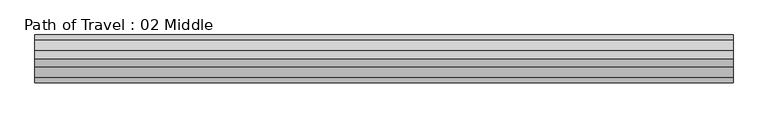
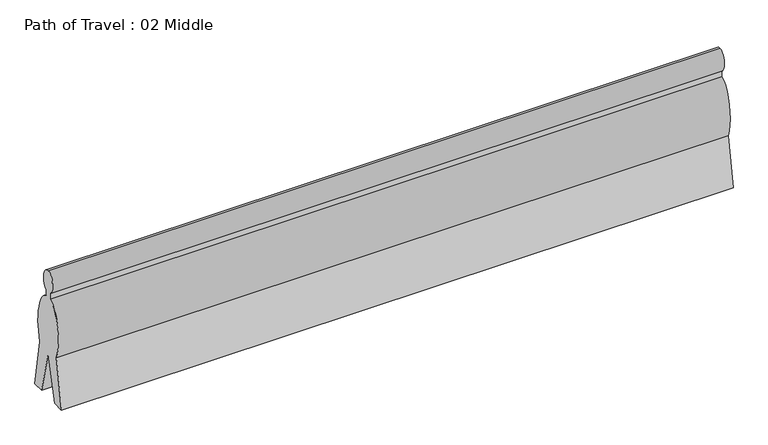
"""IFC4 building model written with IfcOpenShell, lengths in millimetres: proxy geometry, Path of Travel : 02 Middle."""

from ifc_helpers import new_model, si_unit, point, frame, origin, place, context, project, spatial, ellipse_curve, trimmed, source, transform, mapped, element, save
from ifc_brep_helpers import plane_surface, extruded_surface, advanced_brep


def path_of_travel_02_middle_3b68c140(model_context):
    return source(origin(), model_context, "Body", "AdvancedBrep", [
        advanced_brep(
        [(227.5554837, 0.0, 1727.2), (227.5554837, 42.9018657, 1436.6534209), (227.5554837, 42.9018657, 1363.4763406), (227.5554837, 184.1186263, 643.4144547), (227.5554837, 297.5699544, 0.0), (227.5554837, 145.6574193, 0.0), (227.5554837, 0.0, 584.2), (227.5554837, -145.6574193, 0.0), (227.5554837, -297.5699544, 0.0), (227.5554837, -184.1186263, 643.4144547), (227.5554837, -42.9018657, 1363.4763406), (227.5554837, -42.9018657, 1436.6534209), (8914.3554837, 0.0, 1727.2), (8914.3554837, -42.9018657, 1436.6534209), (8914.3554837, -42.9018657, 1363.4763406), (8914.3554837, -184.1186263, 643.4144547), (8914.3554837, -297.5699544, 0.0), (8914.3554837, -145.6574193, 0.0), (8914.3554837, 0.0, 584.2), (8914.3554837, 145.6574193, 0.0), (8914.3554837, 297.5699544, 0.0), (8914.3554837, 184.1186263, 643.4144547), (8914.3554837, 42.9018657, 1363.4763406), (8914.3554837, 42.9018657, 1436.6534209)],
        [
            (0, 1, ellipse_curve(frame((227.5554837, 0.0, 1574.8), z_axis=(-1.0, 0.0, 0.0), x_axis=(0.0, 0.0, 1.0)), 152.4, 101.6)),
            (1, 2),
            (2, 3, ellipse_curve(frame((227.5554837, 0.0, 914.4), z_axis=(-1.0, 0.0, 0.0), x_axis=(0.0, 0.0, -1.0)), 457.2, 228.6)),
            (3, 4),
            (4, 5),
            (5, 6),
            (6, 7),
            (7, 8),
            (8, 9),
            (9, 10, ellipse_curve(frame((227.5554837, 0.0, 914.4), z_axis=(-1.0, 0.0, 0.0), x_axis=(0.0, 0.0, -1.0)), 457.2, 228.6)),
            (10, 11),
            (11, 0, ellipse_curve(frame((227.5554837, 0.0, 1574.8), z_axis=(-1.0, 0.0, 0.0), x_axis=(0.0, 0.0, 1.0)), 152.4, 101.6)),
            (12, 13, ellipse_curve(frame((8914.3554837, 0.0, 1574.8), z_axis=(1.0, 0.0, 0.0), x_axis=(0.0, 0.0, 1.0)), 152.4, 101.6)),
            (13, 14),
            (14, 15, ellipse_curve(frame((8914.3554837, 0.0, 914.4), z_axis=(1.0, 0.0, 0.0), x_axis=(0.0, 0.0, -1.0)), 457.2, 228.6)),
            (15, 16),
            (16, 17),
            (17, 18),
            (18, 19),
            (19, 20),
            (20, 21),
            (21, 22, ellipse_curve(frame((8914.3554837, 0.0, 914.4), z_axis=(1.0, 0.0, 0.0), x_axis=(0.0, 0.0, -1.0)), 457.2, 228.6)),
            (22, 23),
            (23, 12, ellipse_curve(frame((8914.3554837, 0.0, 1574.8), z_axis=(1.0, 0.0, 0.0), x_axis=(0.0, 0.0, 1.0)), 152.4, 101.6)),
            (0, 12),
            (23, 1),
            (22, 2),
            (21, 3),
            (20, 4),
            (19, 5),
            (18, 6),
            (17, 7),
            (16, 8),
            (15, 9),
            (14, 10),
            (13, 11),
        ],
        [
            plane_surface(frame((227.5554837, 0.0, 0.0), z_axis=(-1.0, 0.0, 0.0), x_axis=(0.0, 0.0, 1.0))),
            plane_surface(frame((8914.3554837, 0.0, 0.0), z_axis=(1.0, 0.0, 0.0), x_axis=(0.0, 0.0, 1.0))),
            extruded_surface(trimmed(ellipse_curve(frame((8914.3554837, 0.0, 1574.8), z_axis=(-1.0, 0.0, 0.0), x_axis=(0.0, 0.0, 1.0)), 152.4, 101.6), [point((8914.3554837, 0.0, 1727.2))], [point((8914.3554837, 42.9018657, 1436.6534209))], True, "CARTESIAN"), (-8686.8, 0.0, 0.0), 8686.8),
            plane_surface(frame((227.5554837, 42.9018657, 1436.6534209), z_axis=(0.0, 1.0, 0.0), x_axis=(1.0, 0.0, 0.0))),
            extruded_surface(trimmed(ellipse_curve(frame((8914.3554837, 0.0, 914.4), z_axis=(-1.0, 0.0, 0.0), x_axis=(0.0, 0.0, -1.0)), 457.2, 228.6), [point((8914.3554837, 42.9018657, 1363.4763406))], [point((8914.3554837, 184.1186263, 643.4144547))], True, "CARTESIAN"), (-8686.8, 0.0, 0.0), 8686.8),
            plane_surface(frame((227.5554837, 184.1186263, 643.4144547), z_axis=(0.0, 0.9848077530122078, 0.17364817766693205), x_axis=(1.0, 0.0, 0.0))),
            plane_surface(frame((227.5554837, 297.5699544, 0.0), z_axis=(0.0, 0.0, -1.0), x_axis=(1.0, 0.0, 0.0))),
            plane_surface(frame((227.5554837, 145.6574193, 0.0), z_axis=(0.0, -0.9702957262760199, -0.2419218955995739), x_axis=(1.0, 0.0, 0.0))),
            plane_surface(frame((227.5554837, 0.0, 584.2), z_axis=(0.0, 0.9702957262759961, -0.24192189559966923), x_axis=(1.0, 0.0, 0.0))),
            plane_surface(frame((227.5554837, -145.6574193, 0.0), z_axis=(0.0, 0.0, -1.0), x_axis=(1.0, 0.0, 0.0))),
            plane_surface(frame((227.5554837, -297.5699544, 0.0), z_axis=(0.0, -0.984807753012208, 0.17364817766693066), x_axis=(1.0, 0.0, 0.0))),
            extruded_surface(trimmed(ellipse_curve(frame((8914.3554837, 0.0, 914.4), z_axis=(-1.0, 0.0, 0.0), x_axis=(0.0, 0.0, -1.0)), 457.2, 228.6), [point((8914.3554837, -184.1186263, 643.4144547))], [point((8914.3554837, -42.9018657, 1363.4763406))], True, "CARTESIAN"), (-8686.8, 0.0, 0.0), 8686.8),
            plane_surface(frame((227.5554837, -42.9018657, 1363.4763406), z_axis=(0.0, -1.0, 0.0), x_axis=(1.0, 0.0, 0.0))),
            extruded_surface(trimmed(ellipse_curve(frame((8914.3554837, 0.0, 1574.8), z_axis=(-1.0, 0.0, 0.0), x_axis=(0.0, 0.0, 1.0)), 152.4, 101.6), [point((8914.3554837, -42.9018657, 1436.6534209))], [point((8914.3554837, 0.0, 1727.2))], True, "CARTESIAN"), (-8686.8, 0.0, 0.0), 8686.8),
        ],
        [
            (0, [[1, 2, 3, 4, 5, 6, 7, 8, 9, 10, 11, 12]]),
            (1, [[13, 14, 15, 16, 17, 18, 19, 20, 21, 22, 23, 24]]),
            (2, [[-1, 25, -24, 26]]),
            (3, [[-2, -26, -23, 27]]),
            (4, [[-3, -27, -22, 28]]),
            (5, [[-4, -28, -21, 29]]),
            (6, [[-5, -29, -20, 30]]),
            (7, [[-6, -30, -19, 31]]),
            (8, [[-7, -31, -18, 32]]),
            (9, [[-8, -32, -17, 33]]),
            (10, [[-9, -33, -16, 34]]),
            (11, [[-10, -34, -15, 35]]),
            (12, [[-11, -35, -14, 36]]),
            (13, [[-12, -36, -13, -25]]),
        ],
    ),
    ])


if __name__ == "__main__":
    model = new_model("IFC4")
    model_context = context("Model", 3, world=origin())
    ifc_project = project(units=[si_unit("LENGTHUNIT", "METRE", prefix="MILLI")], contexts=[model_context])
    site = spatial("IfcSite", under=ifc_project)
    building = spatial("IfcBuilding", under=site)
    placement = place(None, origin())
    path_of_travel_02_middle_shape = path_of_travel_02_middle_3b68c140(model_context)
    element("IfcBuildingElementProxy", 1, Name="Path of Travel : 02 Middle", ObjectType="Path of Travel : 02 Middle", at=placement, inside=building, context=model_context, shape_type="MappedRepresentation", body=[
        mapped(path_of_travel_02_middle_shape, transform((0.0, 0.0, 0.0), x_axis=(1.0, 0.0, 0.0), y_axis=(0.0, 1.0, 0.0), z_axis=(0.0, 0.0, 1.0))),
    ])
    save(model, "model.ifc")

# Revit data of these elements
# Type "Path of Travel : 02 Middle"
#   Path of Egress [instance default] = 4' - 0"
#   built-in parameter 1001306 [instance default] = 4 (stored number, unit not read)
#   Dot at Start = no
#   Arrow in Middle = yes
#   Arrow at End = no
#   Egress Path = none
# Element 1 (IfcBuildingElementProxy, "Path of Travel : 02 Middle")
#   Path of Egress = 28' - 6"
#   built-in parameter 1001306 = 28.5 (stored number, unit not read)
#   Materials on its faces: "Egress Path Solid"
# Materials
#   "Egress Path Solid": class "Unassigned", colour RGB 255 128 64, transparency 0.75, Comments = "Rendering appearance not upgraded "
